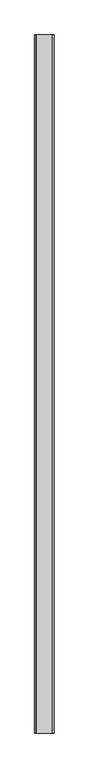
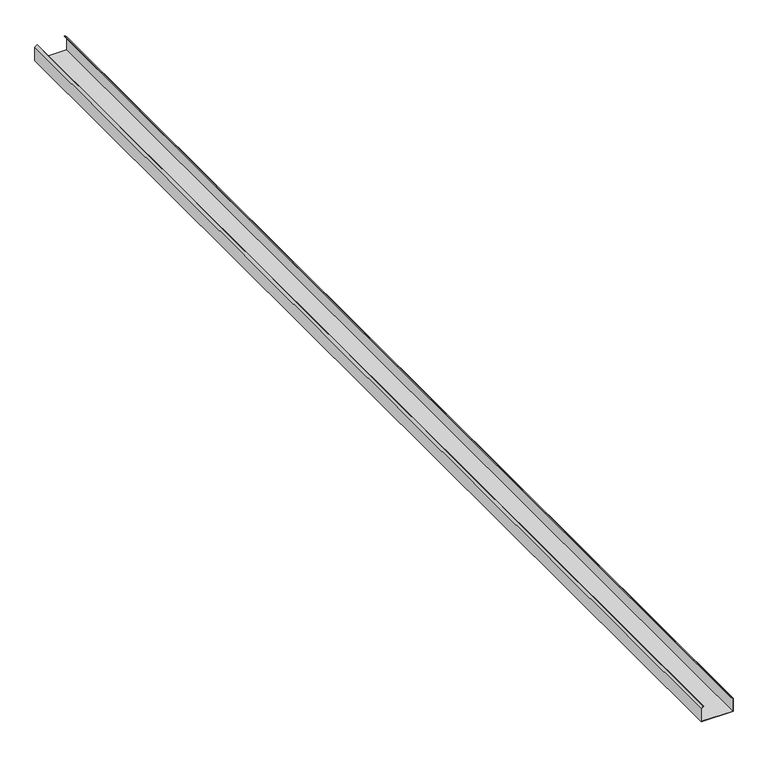
"""IFC4 building model written with IfcOpenShell, lengths in millimetres: proxy geometry, Generic Models 7:Generic Models 1:1:Generic Models 1:1 : Generic Models 7:Generic Models 1:337419:48 : Generic Models 7:Generic Models 1:1:Generic Models 1:1 : Generic Models 7:Generic Models 1:337419:306201."""

from ifc_helpers import new_model, si_unit, frame, origin, place, context, project, spatial, polyline, outline, extrude, source, transform, mapped, element, save


def generic_models_a097da85(model_context):
    return source(origin(), model_context, "Body", "SweptSolid", [
        extrude(outline(polyline([(2446.5359375, 560568.8617239), (2535.4359375, 560568.8617239), (2547.6810414, 560554.2685773), (2545.5528742, 560552.482833), (2534.1404765, 560566.0835989), (2449.3140625, 560566.0835989), (2449.3140625, 560368.4398489), (2534.1404765, 560368.4398489), (2545.5528742, 560382.0406149), (2547.6810414, 560380.2548706), (2535.4359375, 560365.6617239), (2446.5359375, 560365.6617239), (2446.5359375, 560568.8617239)])), frame((0.0, -550498.7163841, 0.0), z_axis=(0.0, 1.0, 0.0), x_axis=(0.0, 0.0, 1.0)), (0.0, 0.0, 1.0), 7315.2),
    ])


if __name__ == "__main__":
    model = new_model("IFC4")
    model_context = context("Model", 3, world=origin())
    ifc_project = project(units=[si_unit("LENGTHUNIT", "METRE", prefix="MILLI")], contexts=[model_context])
    site = spatial("IfcSite", under=ifc_project)
    building = spatial("IfcBuilding", under=site)
    placement = place(None, origin())
    generic_models_shape = generic_models_a097da85(model_context)
    element("IfcBuildingElementProxy", 1, Name="Generic Models 7:Generic Models 1:1:Generic Models 1:1 : Generic Models 7:Generic Models 1:337419:48 : Generic Models 7:Generic Models 1:1:Generic Models 1:1 : Generic Models 7:Generic Models 1:337419:306201", ObjectType="Generic Models 7:Generic Models 1:1:Generic Models 1:1 : Generic Models 7:Generic Models 1:337419:48 : Generic Models 7:Generic Models 1:1:Generic Models 1:1 : Generic Models 7:Generic Models 1:337419:306201", at=placement, inside=building, context=model_context, shape_type="MappedRepresentation", body=[
        mapped(generic_models_shape, transform((0.0, 0.0, 0.0), x_axis=(1.0, 0.0, 0.0), y_axis=(0.0, 1.0, 0.0), z_axis=(0.0, 0.0, 1.0))),
    ])
    save(model, "model.ifc")

# Revit data of these elements
# Type "Generic Models 7:Generic Models 1:1:Generic Models 1:1 : Generic Models 7:Generic Models 1:337419:48 : Generic Models 7:Generic Models 1:1:Generic Models 1:1 : Generic Models 7:Generic Models 1:337419:306201"
#   NameOverride = "Generic Models 7:Generic Models 1:1:Generic Models 1:1 : Generic Models 7:Generic Models 1:337419:306201"
#   ObjectTypeOverride = "Generic Models 1:1 : Generic Models 7:Generic Models 1:337419"
#   Reference = "Generic Models 1"
#   Tag = "306201"
# Element 1 (IfcBuildingElementProxy, "Generic Models 7:Generic Models 1:1:Generic Models 1:1 : Generic Models 7:Generic Models 1:337419:48 : Generic Models 7:Generic Models 1:1:Generic Models 1:1 : Generic Models 7:Generic Models 1:337419:306201")
#   Materials on its faces: "CEE' SECTION (8.0x3.5C - SEE STRUCT. DWGS)"
# Materials
#   "CEE' SECTION (8.0x3.5C - SEE STRUCT. DWGS)": class "Unassigned", colour RGB 210 209 208, transparency 0, Keynote = "M05121300.02", Cost = 0
